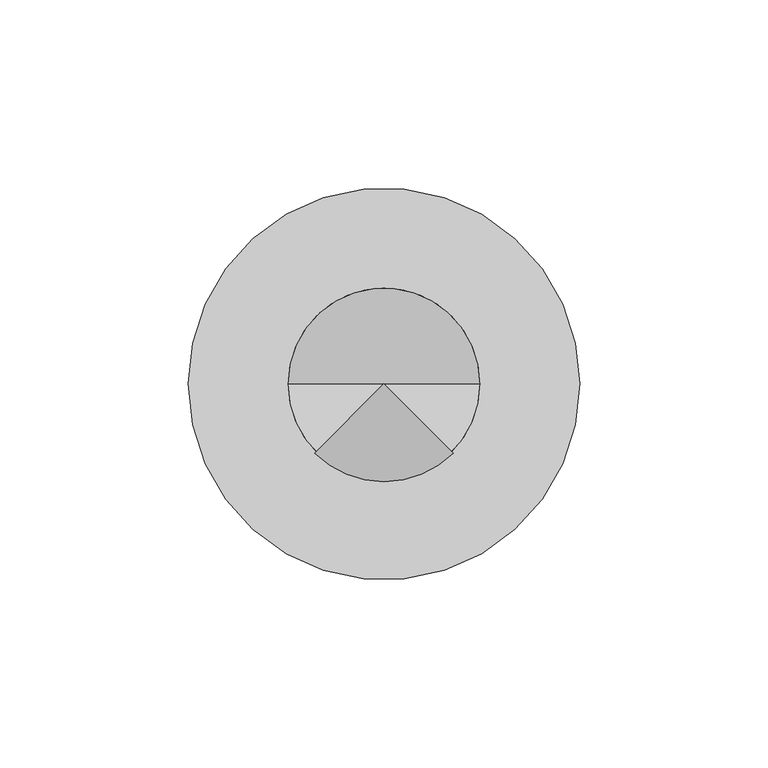
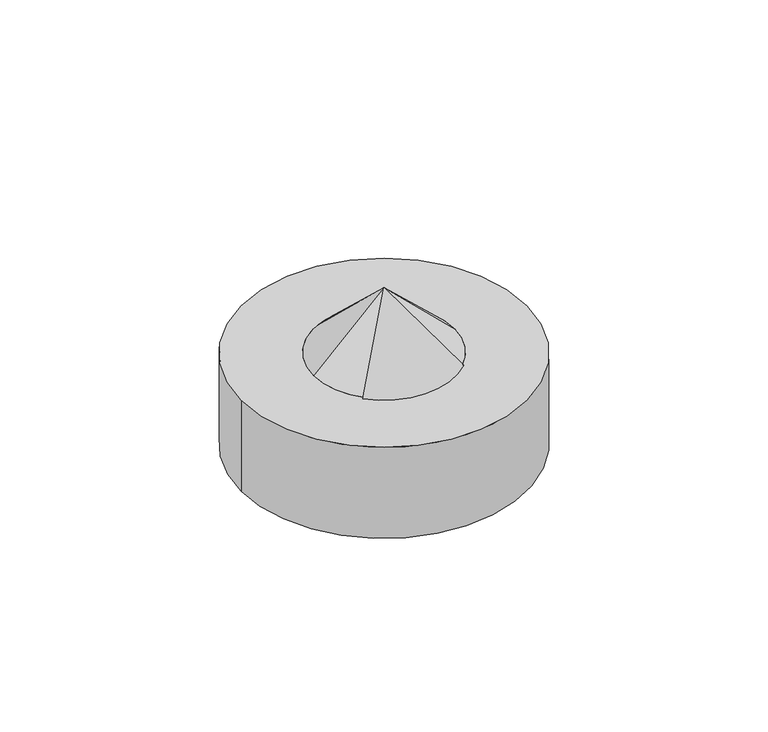
"""IFC4 building model written with IfcOpenShell, lengths in millimetres: alarm geometry, 电子感温探测器 : 防爆型."""

from ifc_helpers import new_model, si_unit, frame, origin, place, context, project, spatial, polyline, circle_curve, source, transform, mapped, element, save
from ifc_brep_helpers import plane_surface, cylinder_surface, revolved_surface, advanced_brep


def alarm_53eb8f19(model_context):
    return source(origin(), model_context, "Body", "AdvancedBrep", [
        advanced_brep(
        [(52.0, 0.0, 0.0), (-52.0, 0.0, 0.0), (52.0, 0.0, 35.0), (-52.0, 0.0, 35.0), (-18.3847763, -18.3847763, 35.0), (0.0, 0.0, 35.0), (18.3847763, -18.3847763, 35.0), (0.0, 0.0, 60.0)],
        [
            (0, 1, circle_curve(frame((0.0, 0.0, 0.0), z_axis=(0.0, 0.0, -1.0), x_axis=(-1.0, 0.0, 0.0)), 52.0)),
            (1, 0, circle_curve(frame((0.0, 0.0, 0.0), z_axis=(0.0, 0.0, -1.0), x_axis=(-1.0, 0.0, 0.0)), 52.0)),
            (2, 3, circle_curve(frame((0.0, 0.0, 35.0), z_axis=(0.0, 0.0, 1.0), x_axis=(-1.0, 0.0, 0.0)), 52.0)),
            (3, 2, circle_curve(frame((0.0, 0.0, 35.0), z_axis=(0.0, 0.0, 1.0), x_axis=(-1.0, 0.0, 0.0)), 52.0)),
            (4, 5),
            (5, 6),
            (6, 4, circle_curve(frame((0.0, 0.0, 35.0), z_axis=(0.0, 0.0, -1.0), x_axis=(-0.7071067811865503, -0.7071067811865446, 0.0)), 26.0)),
            (1, 3),
            (2, 0),
            (4, 7),
            (7, 5),
            (7, 6),
        ],
        [
            plane_surface(frame((-52.0, 0.0, 0.0), z_axis=(0.0, 0.0, -1.0), x_axis=(0.0, 1.0, 0.0))),
            plane_surface(frame((-52.0, 0.0, 35.0), z_axis=(0.0, 0.0, 1.0), x_axis=(0.0, -1.0, 0.0))),
            cylinder_surface(frame((0.0, 0.0, 0.0), z_axis=(0.0, 0.0, 1.0), x_axis=(-1.0, 0.0, 0.0)), 52.0),
            plane_surface(frame((0.0, 0.0, 2609.0581012), z_axis=(-0.7071067811865447, 0.7071067811865505, 0.0), x_axis=(-0.7071067811865505, -0.7071067811865447, 0.0))),
            plane_surface(frame((0.0, 0.0, 2609.0581012), z_axis=(0.7071067811865515, 0.7071067811865437, 0.0), x_axis=(0.7071067811865437, -0.7071067811865515, 0.0))),
            revolved_surface(polyline([(-18.3847763, -18.3847763, 35.0), (0.0, 0.0, 60.0)]), (0.0, 0.0, 2609.0581012), (0.0, 0.0, 1.0)),
        ],
        [
            (0, [[1, 2]]),
            (1, [[3, 4], [5, 6, 7]]),
            (2, [[-2, 8, -3, 9]]),
            (2, [[-1, -9, -4, -8]]),
            (3, [[10, 11, -5]]),
            (4, [[-11, 12, -6]]),
            (5, [[-10, -7, -12]]),
        ],
    ),
        advanced_brep(
        [(26.0, 0.0, 35.0), (-26.0, 0.0, 35.0), (0.0, 0.0, 60.0), (0.0, 0.0, 35.0)],
        [
            (0, 1, circle_curve(frame((0.0, 0.0, 35.0), z_axis=(0.0, 0.0, 1.0), x_axis=(-1.0, 0.0, 0.0)), 26.0)),
            (1, 2),
            (2, 0),
            (1, 0, circle_curve(frame((0.0, 0.0, 35.0), z_axis=(0.0, 0.0, 1.0), x_axis=(-1.0, 0.0, 0.0)), 26.0)),
            (3, 1),
            (0, 3),
        ],
        [
            revolved_surface(polyline([(0.0, 0.0, 60.0), (-26.0, 0.0, 35.0)]), (0.0, 0.0, 2609.0581012), (0.0, 0.0, -1.0)),
            plane_surface(frame((0.0, 0.0, 35.0), z_axis=(0.0, 0.0, -1.0), x_axis=(-1.0, 0.0, 0.0))),
        ],
        [
            (0, [[1, 2, 3]]),
            (0, [[4, -3, -2]]),
            (1, [[5, -1, 6]]),
            (1, [[-6, -4, -5]]),
        ],
    ),
        advanced_brep(
        [(0.0, 0.0, 60.0), (-18.3847763, 18.3847763, 35.0), (0.0, 0.0, 35.0), (18.3847763, 18.3847763, 35.0)],
        [
            (0, 1),
            (1, 2),
            (2, 0),
            (2, 3),
            (3, 0),
            (1, 3, circle_curve(frame((0.0, 0.0, 35.0), z_axis=(0.0, 0.0, -1.0), x_axis=(-0.707106781186547, 0.7071067811865482, 0.0)), 26.0)),
        ],
        [
            plane_surface(frame((0.0, 0.0, 2343.8067943), z_axis=(-0.7071067811865482, -0.707106781186547, 0.0), x_axis=(-0.707106781186547, 0.7071067811865482, 0.0))),
            plane_surface(frame((0.0, 0.0, 2343.8067943), z_axis=(0.7071067811865482, -0.707106781186547, 0.0), x_axis=(0.707106781186547, 0.7071067811865482, 0.0))),
            plane_surface(frame((0.0, 0.0, 35.0), z_axis=(0.0, 0.0, -1.0000000000000002), x_axis=(-0.707106781186547, 0.7071067811865482, 0.0))),
            revolved_surface(polyline([(-18.3847763, 18.3847763, 35.0), (0.0, 0.0, 60.0)]), (0.0, 0.0, 2343.8067943), (0.0, 0.0, 1.0)),
        ],
        [
            (0, [[1, 2, 3]]),
            (1, [[4, 5, -3]]),
            (2, [[-2, 6, -4]]),
            (3, [[-6, -1, -5]]),
        ],
    ),
        advanced_brep(
        [(0.0, 0.0, 60.0), (0.0, 0.0, 35.0), (-18.3847763, 18.3847763, 35.0), (-18.3847763, -18.3847763, 35.0)],
        [
            (0, 1),
            (1, 2),
            (2, 0),
            (0, 3),
            (3, 1),
            (3, 2, circle_curve(frame((0.0, 0.0, 35.0), z_axis=(0.0, 0.0, -1.0), x_axis=(-0.707106781186547, 0.7071067811865482, 0.0)), 26.0)),
        ],
        [
            plane_surface(frame((0.0, 0.0, 2343.8067943), z_axis=(0.7071067811865482, 0.707106781186547, 0.0), x_axis=(-0.707106781186547, 0.7071067811865482, 0.0))),
            plane_surface(frame((0.0, 0.0, 2343.8067943), z_axis=(0.7071067811865459, -0.7071067811865491, 0.0), x_axis=(-0.7071067811865491, -0.7071067811865459, 0.0))),
            plane_surface(frame((0.0, 0.0, 35.0), z_axis=(0.0, 0.0, -1.0000000000000002), x_axis=(-0.707106781186547, 0.7071067811865482, 0.0))),
            revolved_surface(polyline([(-18.3847763, 18.3847763, 35.0), (0.0, 0.0, 60.0)]), (0.0, 0.0, 2343.8067943), (0.0, 0.0, 1.0)),
        ],
        [
            (0, [[1, 2, 3]]),
            (1, [[4, 5, -1]]),
            (2, [[6, -2, -5]]),
            (3, [[-3, -6, -4]]),
        ],
    ),
        advanced_brep(
        [(18.3847763, -18.3847763, 35.0), (0.0, 0.0, 60.0), (0.0, 0.0, 35.0), (18.3847763, 18.3847763, 35.0)],
        [
            (0, 1),
            (1, 2),
            (2, 0),
            (3, 2),
            (1, 3),
            (0, 3, circle_curve(frame((0.0, 0.0, 35.0), z_axis=(0.0, 0.0, 1.0), x_axis=(0.7071067811865503, -0.7071067811865446, 0.0)), 26.0)),
        ],
        [
            plane_surface(frame((0.0, 0.0, 2609.0581012), z_axis=(-0.7071067811865447, -0.7071067811865505, 0.0), x_axis=(0.7071067811865505, -0.7071067811865447, 0.0))),
            plane_surface(frame((0.0, 0.0, 2609.0581012), z_axis=(-0.7071067811865491, 0.707106781186546, 0.0), x_axis=(0.707106781186546, 0.7071067811865491, 0.0))),
            revolved_surface(polyline([(0.0, 0.0, 60.0), (18.3847763, -18.3847763, 35.0)]), (0.0, 0.0, 2609.0581012), (0.0, 0.0, -1.0)),
            plane_surface(frame((0.0, 0.0, 35.0), z_axis=(0.0, 0.0, -1.0), x_axis=(0.7071067811865505, -0.7071067811865447, 0.0))),
        ],
        [
            (0, [[1, 2, 3]]),
            (1, [[4, -2, 5]]),
            (2, [[-1, 6, -5]]),
            (3, [[-6, -3, -4]]),
        ],
    ),
    ])


if __name__ == "__main__":
    model = new_model("IFC4")
    model_context = context("Model", 3, world=origin())
    ifc_project = project(units=[si_unit("LENGTHUNIT", "METRE", prefix="MILLI")], contexts=[model_context])
    site = spatial("IfcSite", under=ifc_project)
    building = spatial("IfcBuilding", under=site)
    placement = place(None, origin())
    alarm_shape = alarm_53eb8f19(model_context)
    element("IfcAlarm", 1, ObjectType="电子感温探测器 : 防爆型", at=placement, inside=building, context=model_context, shape_type="MappedRepresentation", body=[
        mapped(alarm_shape, transform((0.0, 0.0, 0.0), x_axis=(1.0, 0.0, 0.0), y_axis=(0.0, 1.0, 0.0), z_axis=(0.0, 0.0, 1.0))),
    ])
    save(model, "model.ifc")

# Revit data of these elements
# Type "电子感温探测器 : 防爆型"
#   半径 2 = 52 mm
#   半径 1 = 26 mm
#   长度 3 = 18.385 mm
#   长度 2 = 22.517 mm
#   长度 1 = 36.77 mm
#   高度 4 = 1.562 mm
#   高度 3 = 17.5 mm
#   高度 2 = 25 mm
#   高度 1 = 35 mm
#   Default Elevation = 1200 mm
#   可见性 1 = no
#   可见性 2 = yes
#   材质 = none
